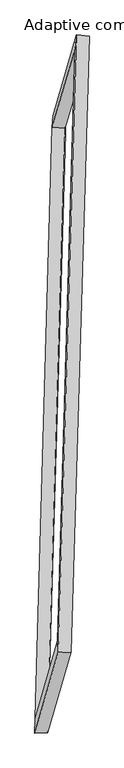
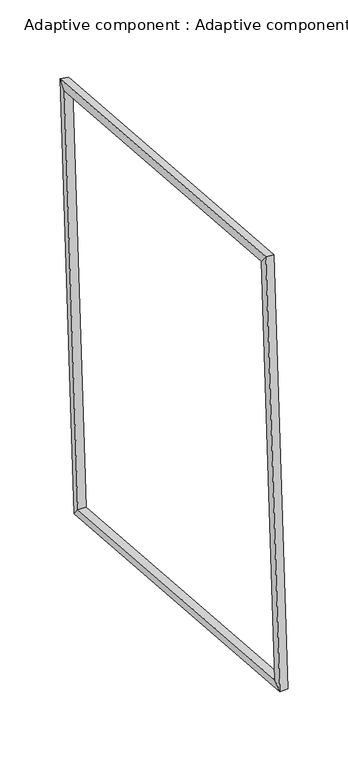
"""IFC4 building model written with IfcOpenShell, lengths in millimetres: proxy geometry, Adaptive component : Adaptive component."""

from ifc_helpers import new_model, si_unit, origin, place, context, project, spatial, faceted_brep, source, transform, mapped, element, save


def adaptive_component_adaptive_component_1b1146f2(model_context):
    return source(origin(), model_context, "Body", "Brep", [
        faceted_brep([(76.1782414, 1246.9137821, 2849.5714254), (140.8162744, 1241.0547977, 2844.6792941), (54.5094187, -1697.7555579, 3186.8612841), (-10.3249612, -1698.5823258, 3192.5318746), (83.6055631, 1318.6933486, 2906.4150071), (-6.6831534, -1755.7022225, 3264.3839357), (148.2435961, 1312.8343641, 2901.5228758), (58.1512265, -1754.8754546, 3258.7133452), (-58.0929472, -2083.6617152, -155.8727019), (-123.1525366, -2085.260312, -156.8877226), (-123.852707, -2157.260856, -213.9324021), (-58.7931175, -2155.6622592, -212.9173814), (28.2139086, 855.1486404, -498.0546919), (-36.649334, 860.235796, -499.8481719), (-33.5639905, 917.1347151, -571.9013308), (31.2992521, 912.0475595, -570.1078508)], [[[0, 1, 2, 3]], [[4, 0, 3, 5]], [[6, 4, 5, 7]], [[1, 6, 7, 2]], [[3, 2, 8, 9]], [[5, 3, 9, 10]], [[7, 5, 10, 11]], [[2, 7, 11, 8]], [[9, 8, 12, 13]], [[10, 9, 13, 14]], [[11, 10, 14, 15]], [[8, 11, 15, 12]], [[13, 12, 1, 0]], [[14, 13, 0, 4]], [[15, 14, 4, 6]], [[12, 15, 6, 1]]]),
    ])


if __name__ == "__main__":
    model = new_model("IFC4")
    model_context = context("Model", 3, world=origin())
    ifc_project = project(units=[si_unit("LENGTHUNIT", "METRE", prefix="MILLI")], contexts=[model_context])
    site = spatial("IfcSite", under=ifc_project)
    building = spatial("IfcBuilding", under=site)
    placement = place(None, origin())
    adaptive_component_adaptive_component_shape = adaptive_component_adaptive_component_1b1146f2(model_context)
    element("IfcBuildingElementProxy", 1, Name="Adaptive component : Adaptive component", ObjectType="Adaptive component : Adaptive component", at=placement, inside=building, context=model_context, shape_type="MappedRepresentation", body=[
        mapped(adaptive_component_adaptive_component_shape, transform((0.0, 0.0, 0.0), x_axis=(1.0, 0.0, 0.0), y_axis=(0.0, 1.0, 0.0), z_axis=(0.0, 0.0, 1.0))),
    ])
    save(model, "model.ifc")

# Revit data of these elements
# Type "Adaptive component : Adaptive component"
#   r [instance default] = 2063.125 mm
#   2r [instance default] = 4126.251 mm
#   Number [instance default] = 5
#   Default Elevation = 0
# Element 1 (IfcBuildingElementProxy, "Adaptive component : Adaptive component")
#   r = 2335.449 mm
#   2r = 4670.898 mm
#   Number = 15
